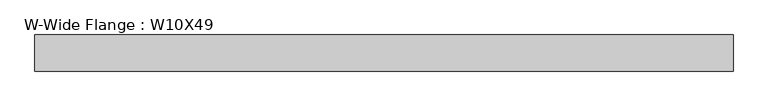
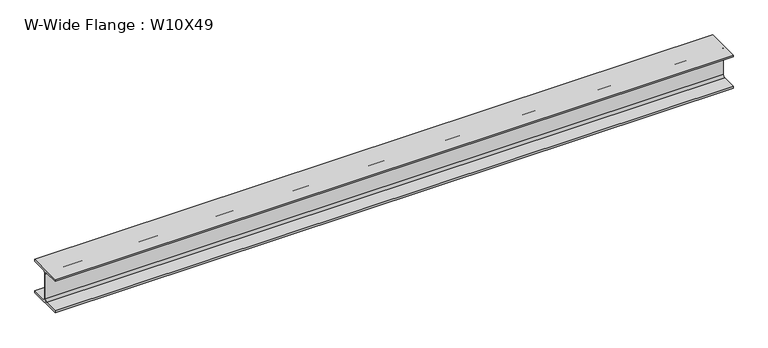
"""IFC4 building model written with IfcOpenShell, lengths in millimetres: beam geometry, W-Wide Flange : W10X49."""

from ifc_helpers import new_model, si_unit, point, frame, frame_2d, origin, place, context, project, spatial, polyline, circle_curve, trimmed, segment, composite_curve, outline, extrude, source, transform, mapped, element, save


def w_wide_flange_w10x49_a7e93ba8(model_context):
    return source(origin(), model_context, "Body", "SweptSolid", [
        extrude(outline(composite_curve([segment(polyline([(127.0, -112.776), (127.0, -127.0), (-127.0, -127.0), (-127.0, -112.776), (-21.844, -112.776)]), True, "CONTINUOUS"), segment(trimmed(circle_curve(frame_2d((-21.844, -95.25)), 17.526), [point((-21.844, -112.776))], [point((-4.318, -95.25))], True, "CARTESIAN"), True, "CONTINUOUS"), segment(polyline([(-4.318, -95.25), (-4.318, 95.25)]), True, "CONTINUOUS"), segment(trimmed(circle_curve(frame_2d((-21.844, 95.25)), 17.526), [point((-4.318, 95.25))], [point((-21.844, 112.776))], True, "CARTESIAN"), True, "CONTINUOUS"), segment(polyline([(-21.844, 112.776), (-127.0, 112.776), (-127.0, 127.0), (127.0, 127.0), (127.0, 112.776), (21.844, 112.776)]), True, "CONTINUOUS"), segment(trimmed(circle_curve(frame_2d((21.844, 95.25)), 17.526), [point((21.844, 112.776))], [point((4.318, 95.25))], True, "CARTESIAN"), True, "CONTINUOUS"), segment(polyline([(4.318, 95.25), (4.318, -95.25)]), True, "CONTINUOUS"), segment(trimmed(circle_curve(frame_2d((21.844, -95.25)), 17.526), [point((4.318, -95.25))], [point((21.844, -112.776))], True, "CARTESIAN"), True, "CONTINUOUS"), segment(polyline([(21.844, -112.776), (127.0, -112.776)]), True, "CONTINUOUS")], self_intersect=False)), frame((-2434.7118235, 0.0, 0.0), z_axis=(1.0, 0.0, 0.0), x_axis=(0.0, 1.0, 0.0)), (0.0, 0.0, 1.0), 4912.4195312),
    ])


if __name__ == "__main__":
    model = new_model("IFC4")
    model_context = context("Model", 3, world=origin())
    ifc_project = project(units=[si_unit("LENGTHUNIT", "METRE", prefix="MILLI")], contexts=[model_context])
    site = spatial("IfcSite", under=ifc_project)
    building = spatial("IfcBuilding", under=site)
    placement = place(None, origin())
    w_wide_flange_w10x49_shape = w_wide_flange_w10x49_a7e93ba8(model_context)
    element("IfcBeam", 1, ObjectType="W-Wide Flange : W10X49", at=placement, inside=building, context=model_context, shape_type="MappedRepresentation", body=[
        mapped(w_wide_flange_w10x49_shape, transform((0.0, 0.0, 0.0), x_axis=(1.0, 0.0, 0.0), y_axis=(0.0, 1.0, 0.0), z_axis=(0.0, 0.0, 1.0))),
    ])
    save(model, "model.ifc")

# Revit data of these elements
# Type "W-Wide Flange : W10X49"
#   Assembly Code = "B10"
#   W = 49
#   Length [instance default] = 1524 mm
#   bf = 254 mm
#   d = 254 mm
#   k = 31.75 mm
#   k2 = 17.526 mm
#   tf = 14.224 mm
#   tw = 8.636 mm
#   A = 0.0092903 m²
#   Structural Material [instance default] = Steel ASTM A992
# Element 1 (IfcBeam, "W-Wide Flange : W10X49")
#   Structural Material = Aluminum, Anodized Red
#   Materials on its faces: "Aluminum, Anodized Red"
# Materials
#   "Steel ASTM A992": class "Metal", colour RGB 128 0 0, transparency 0, Description = "Structural steel 50ksi", Cost = 0
#   "Aluminum, Anodized Red": class "Metal", colour RGB 120 120 120, transparency 0, Description = "Anodized aluminum, red", Cost = 0
